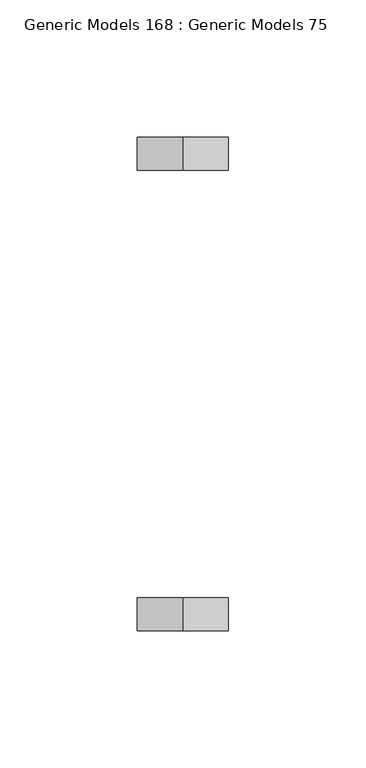
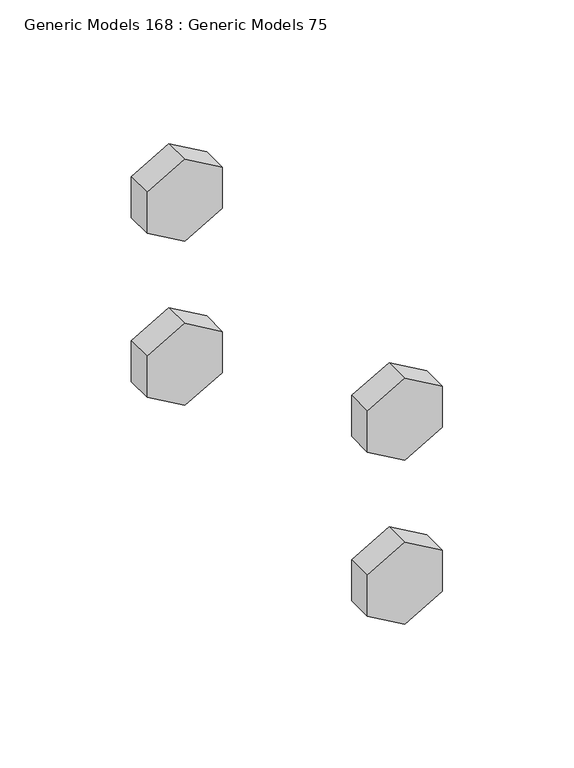
"""IFC4 building model written with IfcOpenShell, lengths in millimetres: proxy geometry, Generic Models 168 : Generic Models 75."""

from ifc_helpers import new_model, si_unit, frame, origin, place, context, project, spatial, polyline, outline, extrude, source, transform, mapped, element, save


def generic_models_168_generic_models_75_f18b7c7c(model_context):
    return source(origin(), model_context, "Body", "SweptSolid", [
        extrude(outline(polyline([(271832.3875, 31991.9073871), (271851.4375, 31991.9073871), (271860.9625, 31975.4096032), (271851.4375, 31958.9118192), (271832.3875, 31958.9118192), (271822.8625, 31975.4096032), (271832.3875, 31991.9073871)])), frame((0.0, 30852.1281612, 0.0), z_axis=(0.0, 1.0, 0.0), x_axis=(0.0, 0.0, 1.0)), (0.0, 0.0, 1.0), 11.90625),
        extrude(outline(polyline([(271756.1875, 31991.9073871), (271775.2375, 31991.9073871), (271784.7625, 31975.4096032), (271775.2375, 31958.9118192), (271756.1875, 31958.9118192), (271746.6625, 31975.4096032), (271756.1875, 31991.9073871)])), frame((0.0, 30852.1281612, 0.0), z_axis=(0.0, 1.0, 0.0), x_axis=(0.0, 0.0, 1.0)), (0.0, 0.0, 1.0), 11.90625),
        extrude(outline(polyline([(271832.3875, 31991.9073871), (271851.4375, 31991.9073871), (271860.9625, 31975.4096032), (271851.4375, 31958.9118192), (271832.3875, 31958.9118192), (271822.8625, 31975.4096032), (271832.3875, 31991.9073871)])), frame((0.0, 30684.6469112, 0.0), z_axis=(0.0, 1.0, 0.0), x_axis=(0.0, 0.0, 1.0)), (0.0, 0.0, 1.0), 11.90625),
        extrude(outline(polyline([(271756.1875, 31991.9073871), (271775.2375, 31991.9073871), (271784.7625, 31975.4096032), (271775.2375, 31958.9118192), (271756.1875, 31958.9118192), (271746.6625, 31975.4096032), (271756.1875, 31991.9073871)])), frame((0.0, 30684.6469112, 0.0), z_axis=(0.0, 1.0, 0.0), x_axis=(0.0, 0.0, 1.0)), (0.0, 0.0, 1.0), 11.90625),
    ])


if __name__ == "__main__":
    model = new_model("IFC4")
    model_context = context("Model", 3, world=origin())
    ifc_project = project(units=[si_unit("LENGTHUNIT", "METRE", prefix="MILLI")], contexts=[model_context])
    site = spatial("IfcSite", under=ifc_project)
    building = spatial("IfcBuilding", under=site)
    placement = place(None, origin())
    generic_models_168_generic_models_75_shape = generic_models_168_generic_models_75_f18b7c7c(model_context)
    element("IfcBuildingElementProxy", 1, Name="Generic Models 168 : Generic Models 75", ObjectType="Generic Models 168 : Generic Models 75", at=placement, inside=building, context=model_context, shape_type="MappedRepresentation", body=[
        mapped(generic_models_168_generic_models_75_shape, transform((0.0, 0.0, 0.0), x_axis=(1.0, 0.0, 0.0), y_axis=(0.0, 1.0, 0.0), z_axis=(0.0, 0.0, 1.0))),
    ])
    save(model, "model.ifc")
